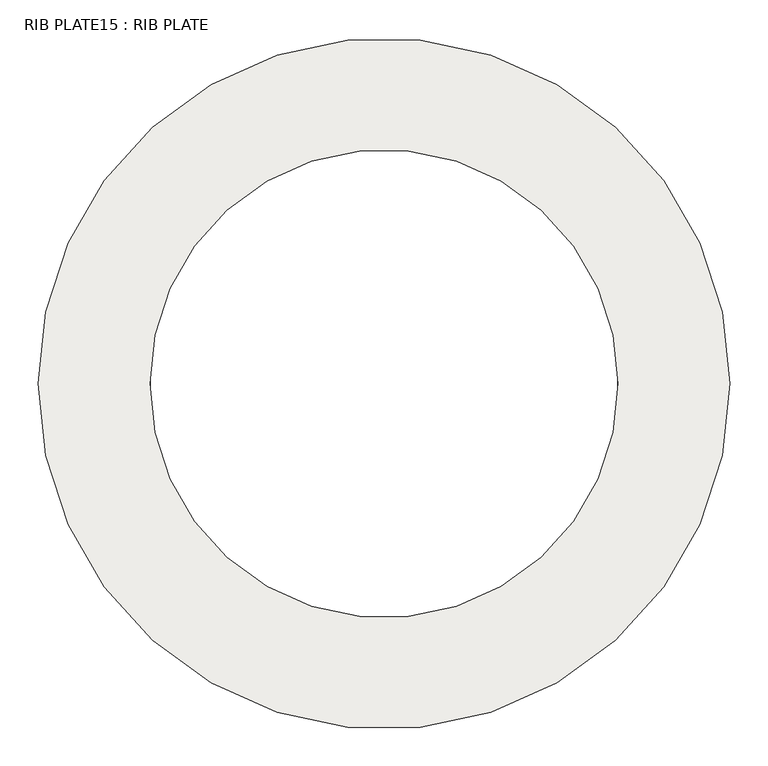
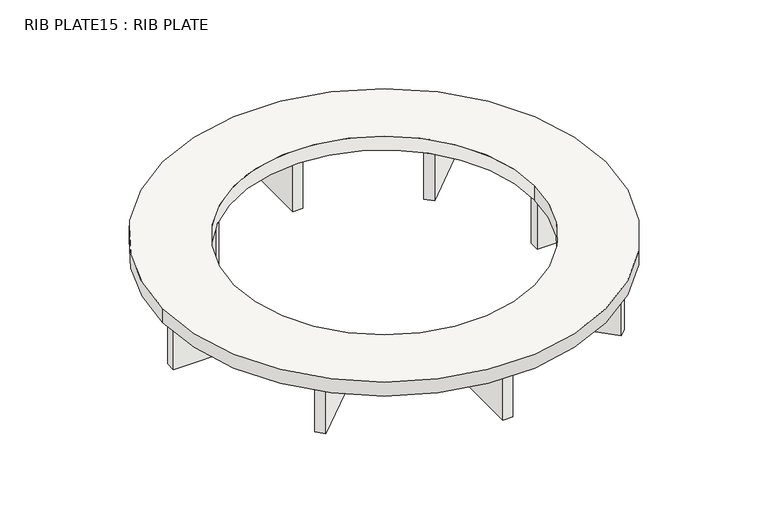
"""IFC4 building model written with IfcOpenShell, lengths in millimetres: slab geometry, RIB PLATE15 : RIB PLATE."""

import ifcopenshell
import ifcopenshell.guid

model = None  # the IFC model being written
_history = None  # IfcOwnerHistory: only IFC2X3 demands one
_inside = {}  # id of a spatial element -> (the spatial element, [elements in it])
_under = {}  # id of a project, library or spatial element -> (it, [spatial elements below it])
_declared = {}  # id of a project -> (the project, [libraries it declares])
_typed = {}  # id of a type object -> (the type object, [elements of that type])
_made_of = {}  # id of a material, layer set ... -> (it, [elements and type objects made of it])


def new_model(schema):
    """Start an empty IFC model of exactly this schema.

    Asked for "IFC4X3", IfcOpenShell would pick the latest addendum, in which some entities
    have other attributes; the version numbers below select the first issue.
    IFC2X3 requires an IfcOwnerHistory on every rooted entity: one is made here for all.
    """
    global model, _history
    if schema == "IFC4X3":
        model = ifcopenshell.file(schema_version=(4, 3, 0, 0))
    else:
        model = ifcopenshell.file(schema=schema)
    _inside.clear()
    _under.clear()
    _declared.clear()
    _typed.clear()
    _made_of.clear()
    _history = None
    if model.schema == "IFC2X3":
        org = make("IfcOrganization", Name="unknown")
        user = make(
            "IfcPersonAndOrganization",
            ThePerson=make("IfcPerson", FamilyName="unknown"),
            TheOrganization=org,
        )
        app = make(
            "IfcApplication",
            ApplicationDeveloper=org,
            Version="unknown",
            ApplicationFullName="unknown",
            ApplicationIdentifier="unknown",
        )
        _history = make(
            "IfcOwnerHistory",
            OwningUser=user,
            OwningApplication=app,
            ChangeAction="ADDED",
            CreationDate=0,
        )
    return model


def make(cls, **values):
    """One entity of the class cls with the attributes given. An attribute that is None is left unset."""
    return model.create_entity(
        cls, **{name: value for name, value in values.items() if value is not None}
    )


def rooted(cls, **values):
    """An entity with a GlobalId (a new one), such as an element, a storey or a relation."""
    return make(cls, GlobalId=ifcopenshell.guid.new(), OwnerHistory=_history, **values)


def si_unit(unit_type, name, prefix=None):
    """IfcSIUnit, for example si_unit("LENGTHUNIT", "METRE", prefix="MILLI")."""
    return make("IfcSIUnit", UnitType=unit_type, Prefix=prefix, Name=name)


def assignment(units):
    """IfcUnitAssignment: the units of a project."""
    return None if units is None else make("IfcUnitAssignment", Units=units)


def point(xyz):
    """IfcCartesianPoint."""
    return None if xyz is None else make("IfcCartesianPoint", Coordinates=xyz)


def direction(xyz):
    """IfcDirection."""
    return None if xyz is None else make("IfcDirection", DirectionRatios=xyz)


def frame(location, z_axis=None, x_axis=None):
    """IfcAxis2Placement3D, a coordinate frame: its origin and axes. An axis left out is left unset."""
    return make(
        "IfcAxis2Placement3D",
        Location=point(location),
        Axis=direction(z_axis),
        RefDirection=direction(x_axis),
    )


def frame_2d(location, x_axis=None):
    """IfcAxis2Placement2D, a coordinate frame in the plane: its origin and x axis."""
    return make(
        "IfcAxis2Placement2D", Location=point(location), RefDirection=direction(x_axis)
    )


def origin():
    """The frame at (0, 0, 0) with its axes left unset."""
    return frame((0.0, 0.0, 0.0))


def place(relative_to, where):
    """IfcLocalPlacement: puts the frame where relative to a parent placement (None: the world)."""
    return make(
        "IfcLocalPlacement", PlacementRelTo=relative_to, RelativePlacement=where
    )


def context(
    kind, dimensions, precision=None, world=None, true_north=None, identifier=None
):
    """IfcGeometricRepresentationContext, for example the 3D "Model" context."""
    return make(
        "IfcGeometricRepresentationContext",
        ContextIdentifier=identifier,
        ContextType=kind,
        CoordinateSpaceDimension=dimensions,
        Precision=precision,
        WorldCoordinateSystem=world,
        TrueNorth=true_north,
    )


def project(units=None, contexts=None):
    """IfcProject with its units and contexts."""
    return rooted(
        "IfcProject",
        Name="project",
        RepresentationContexts=contexts,
        UnitsInContext=assignment(units),
    )


def spatial(cls, under=None, at=None, **own):
    """A site, building, storey or space (cls), placed at a placement, below another one or the project."""
    s = rooted(cls, ObjectPlacement=at, **own)
    if under is not None:
        _under.setdefault(under.id(), (under, []))[1].append(s)
    return s


def polyline(points):
    """IfcPolyline through the points."""
    return make("IfcPolyline", Points=[point(p) for p in points])


def circle_curve(where, radius):
    """IfcCircle in the frame where."""
    return make("IfcCircle", Position=where, Radius=radius)


def trimmed(basis, trim1, trim2, sense, master):
    """IfcTrimmedCurve: the piece of a basis curve between two trims."""
    return make(
        "IfcTrimmedCurve",
        BasisCurve=basis,
        Trim1=trim1,
        Trim2=trim2,
        SenseAgreement=sense,
        MasterRepresentation=master,
    )


def segment(curve, same_sense, transition):
    """IfcCompositeCurveSegment."""
    return make(
        "IfcCompositeCurveSegment",
        Transition=transition,
        SameSense=same_sense,
        ParentCurve=curve,
    )


def composite_curve(segments, self_intersect=None):
    """IfcCompositeCurve: segments joined end to end."""
    return make("IfcCompositeCurve", Segments=segments, SelfIntersect=self_intersect)


def outline(outer, holes=None, kind="AREA"):
    """IfcArbitraryClosedProfileDef: a profile drawn as a closed curve; with holes, ...WithVoids."""
    if holes is None:
        return make("IfcArbitraryClosedProfileDef", ProfileType=kind, OuterCurve=outer)
    return make(
        "IfcArbitraryProfileDefWithVoids",
        ProfileType=kind,
        OuterCurve=outer,
        InnerCurves=holes,
    )


def extrude(swept, where, along, depth):
    """IfcExtrudedAreaSolid: the profile swept, set in the frame where, extruded along a direction by depth."""
    return make(
        "IfcExtrudedAreaSolid",
        SweptArea=swept,
        Position=where,
        ExtrudedDirection=direction(along),
        Depth=depth,
    )


def shape(context_of_items, identifier, shape_type, items):
    """IfcShapeRepresentation: the items that make up one representation, for example the "Body"."""
    return make(
        "IfcShapeRepresentation",
        ContextOfItems=context_of_items,
        RepresentationIdentifier=identifier,
        RepresentationType=shape_type,
        Items=items,
    )


def source(mapping_origin, context_of_items, identifier, shape_type, items):
    """IfcRepresentationMap: a shape defined once, which mapped items show again and again."""
    return make(
        "IfcRepresentationMap",
        MappingOrigin=mapping_origin,
        MappedRepresentation=shape(context_of_items, identifier, shape_type, items),
    )


def transform(
    local_origin,
    x_axis=None,
    y_axis=None,
    z_axis=None,
    scale=None,
    scale2=None,
    scale3=None,
    uniform=True,
):
    """IfcCartesianTransformationOperator3D, or its non-uniform kind. x_axis, y_axis, z_axis: its Axis1, 2, 3."""
    if uniform:
        return make(
            "IfcCartesianTransformationOperator3D",
            Axis1=direction(x_axis),
            Axis2=direction(y_axis),
            LocalOrigin=point(local_origin),
            Scale=scale,
            Axis3=direction(z_axis),
        )
    return make(
        "IfcCartesianTransformationOperator3DnonUniform",
        Axis1=direction(x_axis),
        Axis2=direction(y_axis),
        LocalOrigin=point(local_origin),
        Scale=scale,
        Axis3=direction(z_axis),
        Scale2=scale2,
        Scale3=scale3,
    )


def mapped(mapping_source, mapping_target):
    """IfcMappedItem: shows the shape of a source again, moved by a transform."""
    return make(
        "IfcMappedItem", MappingSource=mapping_source, MappingTarget=mapping_target
    )


def made_of(thing, what):
    """Note that an element or type object is made of a material, layer set ...; save() writes the relation."""
    if what is not None:
        _made_of.setdefault(what.id(), (what, []))[1].append(thing)
    return thing


def element(
    cls,
    number,
    at=None,
    inside=None,
    cuts=None,
    type_object=None,
    material=None,
    context=None,
    identifier="Body",
    shape_type=None,
    held_by="IfcProductDefinitionShape",
    body=None,
    shapes=None,
    **own,
):
    """One element of the class cls, such as IfcWall. Its Tag is "e" and its number.

    at: its placement. inside: the storey or other place that contains it. cuts: it is an
    opening in that element (IfcRelVoidsElement). A single representation is given by context,
    identifier, shape_type and body (its items); several are given by shapes. held_by: the class
    of the entity that holds the representations. save() writes the other relations.
    """
    e = rooted(cls, Tag="e%d" % number, ObjectPlacement=at, **own)
    if body is not None:
        shapes = [shape(context, identifier, shape_type, body)]
    if shapes is not None:
        e.Representation = make(held_by, Representations=shapes)
    if inside is not None:
        _inside.setdefault(inside.id(), (inside, []))[1].append(e)
    if cuts is not None:
        rooted(
            "IfcRelVoidsElement", RelatingBuildingElement=cuts, RelatedOpeningElement=e
        )
    if type_object is not None:
        _typed.setdefault(type_object.id(), (type_object, []))[1].append(e)
    return made_of(e, material)


def aggregate(whole, parts):
    """IfcRelAggregates: a whole, such as a stair, and the parts it consists of."""
    return rooted("IfcRelAggregates", RelatingObject=whole, RelatedObjects=parts)


def save(model, path):
    """Write the relations noted so far, then the file.

    IfcRelAggregates (storeys below a building ...), IfcRelContainedInSpatialStructure (elements
    in a storey), IfcRelDefinesByType, IfcRelAssociatesMaterial and IfcRelDeclares: one each for
    every whole, place, type object, material and project.
    """
    for whole, parts in _under.values():
        aggregate(whole, parts)
    for where, things in _inside.values():
        rooted(
            "IfcRelContainedInSpatialStructure",
            RelatedElements=things,
            RelatingStructure=where,
        )
    for kind, things in _typed.values():
        rooted("IfcRelDefinesByType", RelatedObjects=things, RelatingType=kind)
    for what, things in _made_of.values():
        rooted("IfcRelAssociatesMaterial", RelatedObjects=things, RelatingMaterial=what)
    for by, libraries in _declared.values():
        rooted("IfcRelDeclares", RelatingContext=by, RelatedDefinitions=libraries)
    model.write(path)


def rib_plate15_rib_plate_fba11e19(model_context):
    return source(origin(), model_context, "Body", "SweptSolid", [
        extrude(outline(composite_curve([segment(trimmed(circle_curve(frame_2d((7920.0, 33979.5208589)), 450.0), [point((7470.0, 33979.5208589))], [point((8370.0, 33979.5208589))], False, "CARTESIAN"), True, "CONTINUOUS"), segment(trimmed(circle_curve(frame_2d((7920.0, 33979.5208589)), 450.0), [point((8370.0, 33979.5208589))], [point((7470.0, 33979.5208589))], False, "CARTESIAN"), True, "CONTINUOUS")], self_intersect=False), holes=[composite_curve([segment(trimmed(circle_curve(frame_2d((7920.0, 33979.5208589)), 304.6641594), [point((7615.3358406, 33979.5208589))], [point((8224.6641594, 33979.5208589))], True, "CARTESIAN"), True, "CONTINUOUS"), segment(trimmed(circle_curve(frame_2d((7920.0, 33979.5208589)), 304.6641594), [point((8224.6641594, 33979.5208589))], [point((7615.3358406, 33979.5208589))], True, "CARTESIAN"), True, "CONTINUOUS")], self_intersect=False)]), frame((0.0, 0.0, -1030.0), z_axis=(0.0, 0.0, 1.0), x_axis=(1.0, 0.0, 0.0)), (0.0, 0.0, 1.0), 30.0),
        extrude(outline(polyline([(8220.1668286, 33665.2118947), (8128.2429471, 33757.1357762), (8142.3850827, 33771.2779118), (8234.3089642, 33679.3540303), (8220.1668286, 33665.2118947)])), frame((0.0, 0.0, -1130.0), z_axis=(0.0, 0.0, 1.0), x_axis=(1.0, 0.0, 0.0)), (0.0, 0.0, 1.0), 100.0),
        extrude(outline(polyline([(8354.5, 33969.5208589), (8224.5, 33969.5208589), (8224.5, 33989.5208589), (8354.5, 33989.5208589), (8354.5, 33969.5208589)])), frame((0.0, 0.0, -1130.0), z_axis=(0.0, 0.0, 1.0), x_axis=(1.0, 0.0, 0.0)), (0.0, 0.0, 1.0), 100.0),
        extrude(outline(polyline([(8234.3089642, 34279.6876875), (8142.3850827, 34187.7638059), (8128.2429471, 34201.9059416), (8220.1668286, 34293.8298231), (8234.3089642, 34279.6876875)])), frame((0.0, 0.0, -1130.0), z_axis=(0.0, 0.0, 1.0), x_axis=(1.0, 0.0, 0.0)), (0.0, 0.0, 1.0), 100.0),
        extrude(outline(polyline([(7930.0, 34414.0208589), (7930.0, 34284.0208589), (7910.0, 34284.0208589), (7910.0, 34414.0208589), (7930.0, 34414.0208589)])), frame((0.0, 0.0, -1130.0), z_axis=(0.0, 0.0, 1.0), x_axis=(1.0, 0.0, 0.0)), (0.0, 0.0, 1.0), 100.0),
        extrude(outline(polyline([(7619.8331714, 34293.8298231), (7711.7570529, 34201.9059416), (7697.6149173, 34187.7638059), (7605.6910358, 34279.6876875), (7619.8331714, 34293.8298231)])), frame((0.0, 0.0, -1130.0), z_axis=(0.0, 0.0, 1.0), x_axis=(1.0, 0.0, 0.0)), (0.0, 0.0, 1.0), 100.0),
        extrude(outline(polyline([(7485.5, 33989.5208589), (7615.5, 33989.5208589), (7615.5, 33969.5208589), (7485.5, 33969.5208589), (7485.5, 33989.5208589)])), frame((0.0, 0.0, -1130.0), z_axis=(0.0, 0.0, 1.0), x_axis=(1.0, 0.0, 0.0)), (0.0, 0.0, 1.0), 100.0),
        extrude(outline(polyline([(7605.6910358, 33679.3540303), (7697.6149173, 33771.2779118), (7711.7570529, 33757.1357762), (7619.8331714, 33665.2118947), (7605.6910358, 33679.3540303)])), frame((0.0, 0.0, -1130.0), z_axis=(0.0, 0.0, 1.0), x_axis=(1.0, 0.0, 0.0)), (0.0, 0.0, 1.0), 100.0),
        extrude(outline(polyline([(7910.0, 33545.0208589), (7910.0, 33675.0208589), (7930.0, 33675.0208589), (7930.0, 33545.0208589), (7910.0, 33545.0208589)])), frame((0.0, 0.0, -1130.0), z_axis=(0.0, 0.0, 1.0), x_axis=(1.0, 0.0, 0.0)), (0.0, 0.0, 1.0), 100.0),
    ])


if __name__ == "__main__":
    model = new_model("IFC4")
    model_context = context("Model", 3, world=origin())
    ifc_project = project(units=[si_unit("LENGTHUNIT", "METRE", prefix="MILLI")], contexts=[model_context])
    site = spatial("IfcSite", under=ifc_project)
    building = spatial("IfcBuilding", under=site)
    placement = place(None, origin())
    rib_plate15_rib_plate_shape = rib_plate15_rib_plate_fba11e19(model_context)
    element("IfcSlab", 1, ObjectType="RIB PLATE15 : RIB PLATE", at=placement, inside=building, context=model_context, shape_type="MappedRepresentation", body=[
        mapped(rib_plate15_rib_plate_shape, transform((0.0, 0.0, 0.0), x_axis=(1.0, 0.0, 0.0), y_axis=(0.0, 1.0, 0.0), z_axis=(0.0, 0.0, 1.0))),
    ])
    save(model, "model.ifc")

# Revit data of these elements
# Element 1 (IfcSlab, "RIB PLATE15 : RIB PLATE")
#   Materials on its faces: "Metal - Steel"
# Materials
#   "Metal - Steel": class "Metal", colour RGB 247 247 247, transparency 0, Cost = 0
